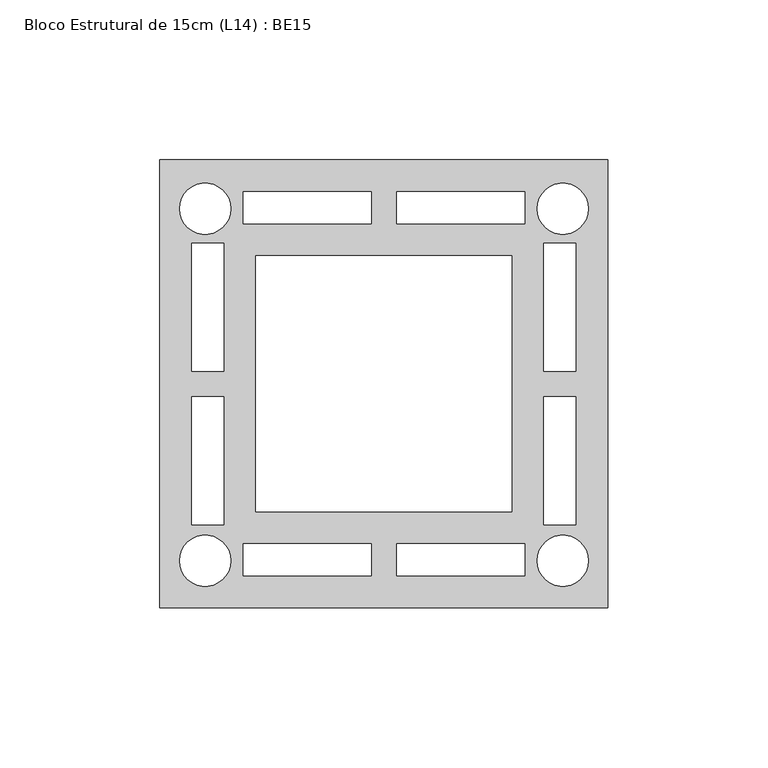
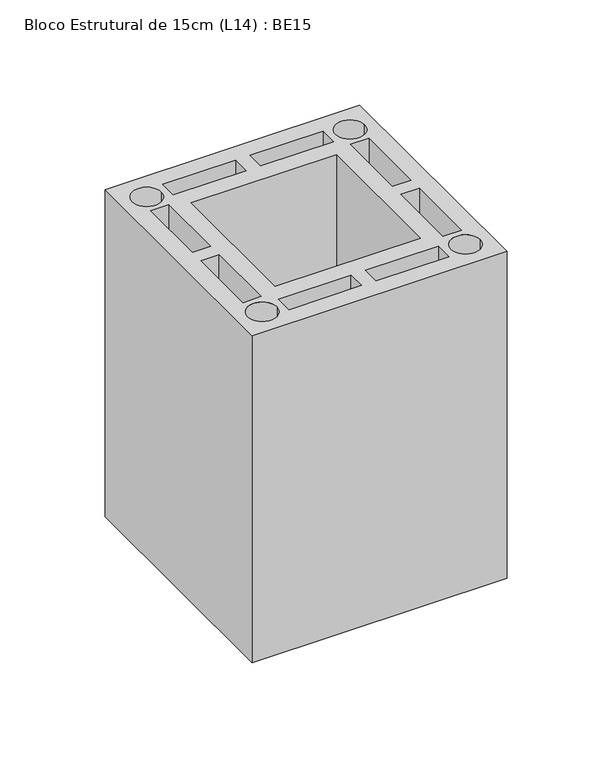
"""IFC4 building model written with IfcOpenShell, lengths in millimetres: proxy geometry, Bloco Estrutural de 15cm (L14) : BE15."""

from ifc_helpers import new_model, si_unit, point, frame_2d, origin, origin_with_axes, place, context, project, spatial, polyline, circle_curve, trimmed, segment, composite_curve, outline, extrude, source, transform, mapped, element, save


def bloco_estrutural_de_15cm_l14_be15_329fd50e(model_context):
    return source(origin(), model_context, "Body", "SweptSolid", [
        extrude(outline(polyline([(0.0, 140.0), (140.0, 140.0), (140.0, 0.0), (0.0, 0.0), (0.0, 140.0)]), holes=[polyline([(30.0, 110.0), (30.0, 30.0), (110.0, 30.0), (110.0, 110.0), (30.0, 110.0)]), composite_curve([segment(trimmed(circle_curve(frame_2d((14.1087523, 124.7509514)), 8.0), [point((6.1087523, 124.7509514))], [point((22.1087523, 124.7509514))], True, "CARTESIAN"), True, "CONTINUOUS"), segment(trimmed(circle_curve(frame_2d((14.1087523, 124.7509514)), 8.0), [point((22.1087523, 124.7509514))], [point((6.1087523, 124.7509514))], True, "CARTESIAN"), True, "CONTINUOUS")], self_intersect=False), composite_curve([segment(trimmed(circle_curve(frame_2d((14.1087523, 14.7509514)), 8.0), [point((6.1087523, 14.7509514))], [point((22.1087523, 14.7509514))], True, "CARTESIAN"), True, "CONTINUOUS"), segment(trimmed(circle_curve(frame_2d((14.1087523, 14.7509514)), 8.0), [point((22.1087523, 14.7509514))], [point((6.1087523, 14.7509514))], True, "CARTESIAN"), True, "CONTINUOUS")], self_intersect=False), polyline([(20.0, 66.0), (10.0, 66.0), (10.0, 26.0), (20.0, 26.0), (20.0, 66.0)]), polyline([(20.0, 74.0), (20.0, 114.0), (10.0, 114.0), (10.0, 74.0), (20.0, 74.0)]), composite_curve([segment(trimmed(circle_curve(frame_2d((125.8912477, 124.7509514)), 8.0), [point((133.8912477, 124.7509514))], [point((117.8912477, 124.7509514))], True, "CARTESIAN"), True, "CONTINUOUS"), segment(trimmed(circle_curve(frame_2d((125.8912477, 124.7509514)), 8.0), [point((117.8912477, 124.7509514))], [point((133.8912477, 124.7509514))], True, "CARTESIAN"), True, "CONTINUOUS")], self_intersect=False), composite_curve([segment(trimmed(circle_curve(frame_2d((125.8912477, 14.7509514)), 8.0), [point((133.8912477, 14.7509514))], [point((117.8912477, 14.7509514))], True, "CARTESIAN"), True, "CONTINUOUS"), segment(trimmed(circle_curve(frame_2d((125.8912477, 14.7509514)), 8.0), [point((117.8912477, 14.7509514))], [point((133.8912477, 14.7509514))], True, "CARTESIAN"), True, "CONTINUOUS")], self_intersect=False), polyline([(120.0, 66.0), (120.0, 26.0), (130.0, 26.0), (130.0, 66.0), (120.0, 66.0)]), polyline([(120.0, 74.0), (130.0, 74.0), (130.0, 114.0), (120.0, 114.0), (120.0, 74.0)]), polyline([(66.0, 120.0), (66.0, 130.0), (26.0, 130.0), (26.0, 120.0), (66.0, 120.0)]), polyline([(74.0, 120.0), (114.0, 120.0), (114.0, 130.0), (74.0, 130.0), (74.0, 120.0)]), polyline([(66.0, 20.0), (26.0, 20.0), (26.0, 10.0), (66.0, 10.0), (66.0, 20.0)]), polyline([(74.0, 20.0), (74.0, 10.0), (114.0, 10.0), (114.0, 20.0), (74.0, 20.0)])]), origin_with_axes(), (0.0, 0.0, 1.0), 190.0),
    ])


if __name__ == "__main__":
    model = new_model("IFC4")
    model_context = context("Model", 3, world=origin())
    ifc_project = project(units=[si_unit("LENGTHUNIT", "METRE", prefix="MILLI")], contexts=[model_context])
    site = spatial("IfcSite", under=ifc_project)
    building = spatial("IfcBuilding", under=site)
    placement = place(None, origin())
    bloco_estrutural_de_15cm_l14_be15_shape = bloco_estrutural_de_15cm_l14_be15_329fd50e(model_context)
    element("IfcBuildingElementProxy", 1, Name="Bloco Estrutural de 15cm (L14) : BE15", ObjectType="Bloco Estrutural de 15cm (L14) : BE15", at=placement, inside=building, context=model_context, shape_type="MappedRepresentation", body=[
        mapped(bloco_estrutural_de_15cm_l14_be15_shape, transform((0.0, 0.0, 0.0), x_axis=(1.0, 0.0, 0.0), y_axis=(0.0, 1.0, 0.0), z_axis=(0.0, 0.0, 1.0))),
    ])
    save(model, "model.ifc")

# Revit data of these elements
# Type "Bloco Estrutural de 15cm (L14) : BE15"
#   Material [instance default] = Blocos Cerâmicos
#   Default Elevation = 0
# Element 1 (IfcBuildingElementProxy, "Bloco Estrutural de 15cm (L14) : BE15")
#   Materials on its faces: "Blocos Cerâmicos"
# Materials
#   "Blocos Cerâmicos": class "Genérico", colour RGB 177 84 47, transparency 0, Cost = 0
